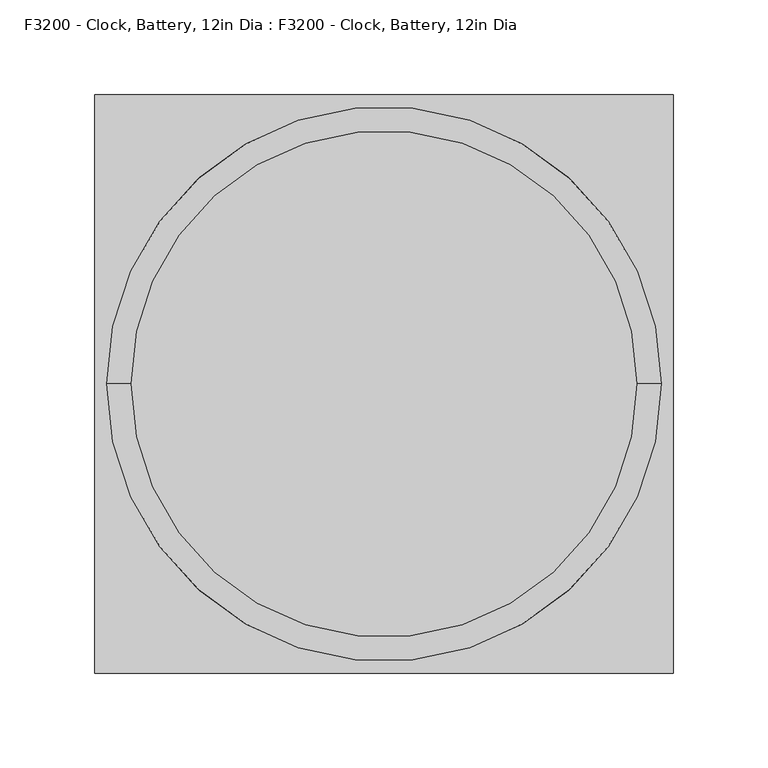
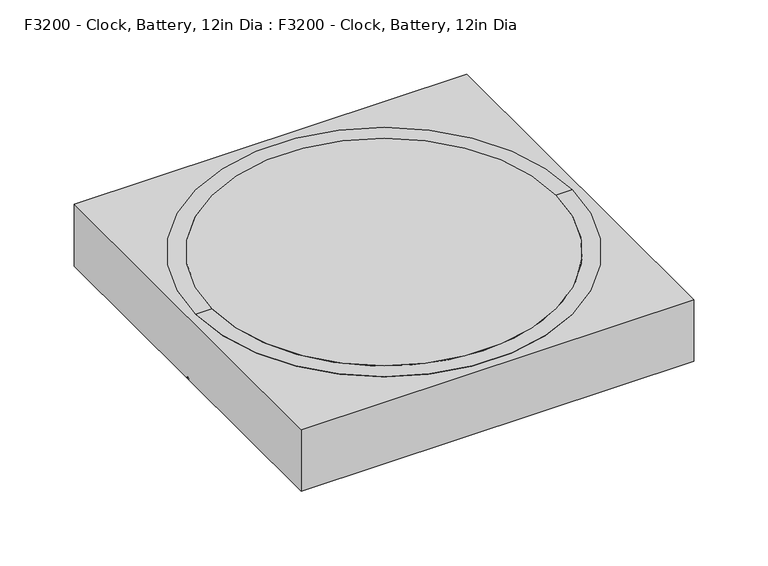
"""IFC4 building model written with IfcOpenShell, lengths in millimetres: proxy geometry, F3200 - Clock, Battery, 12in Dia : F3200 - Clock, Battery, 12in Dia."""

import ifcopenshell
import ifcopenshell.guid

model = None  # the IFC model being written
_history = None  # IfcOwnerHistory: only IFC2X3 demands one
_inside = {}  # id of a spatial element -> (the spatial element, [elements in it])
_under = {}  # id of a project, library or spatial element -> (it, [spatial elements below it])
_declared = {}  # id of a project -> (the project, [libraries it declares])
_typed = {}  # id of a type object -> (the type object, [elements of that type])
_made_of = {}  # id of a material, layer set ... -> (it, [elements and type objects made of it])


def new_model(schema):
    """Start an empty IFC model of exactly this schema.

    Asked for "IFC4X3", IfcOpenShell would pick the latest addendum, in which some entities
    have other attributes; the version numbers below select the first issue.
    IFC2X3 requires an IfcOwnerHistory on every rooted entity: one is made here for all.
    """
    global model, _history
    if schema == "IFC4X3":
        model = ifcopenshell.file(schema_version=(4, 3, 0, 0))
    else:
        model = ifcopenshell.file(schema=schema)
    _inside.clear()
    _under.clear()
    _declared.clear()
    _typed.clear()
    _made_of.clear()
    _history = None
    if model.schema == "IFC2X3":
        org = make("IfcOrganization", Name="unknown")
        user = make(
            "IfcPersonAndOrganization",
            ThePerson=make("IfcPerson", FamilyName="unknown"),
            TheOrganization=org,
        )
        app = make(
            "IfcApplication",
            ApplicationDeveloper=org,
            Version="unknown",
            ApplicationFullName="unknown",
            ApplicationIdentifier="unknown",
        )
        _history = make(
            "IfcOwnerHistory",
            OwningUser=user,
            OwningApplication=app,
            ChangeAction="ADDED",
            CreationDate=0,
        )
    return model


def make(cls, **values):
    """One entity of the class cls with the attributes given. An attribute that is None is left unset."""
    return model.create_entity(
        cls, **{name: value for name, value in values.items() if value is not None}
    )


def rooted(cls, **values):
    """An entity with a GlobalId (a new one), such as an element, a storey or a relation."""
    return make(cls, GlobalId=ifcopenshell.guid.new(), OwnerHistory=_history, **values)


def si_unit(unit_type, name, prefix=None):
    """IfcSIUnit, for example si_unit("LENGTHUNIT", "METRE", prefix="MILLI")."""
    return make("IfcSIUnit", UnitType=unit_type, Prefix=prefix, Name=name)


def assignment(units):
    """IfcUnitAssignment: the units of a project."""
    return None if units is None else make("IfcUnitAssignment", Units=units)


def point(xyz):
    """IfcCartesianPoint."""
    return None if xyz is None else make("IfcCartesianPoint", Coordinates=xyz)


def direction(xyz):
    """IfcDirection."""
    return None if xyz is None else make("IfcDirection", DirectionRatios=xyz)


def frame(location, z_axis=None, x_axis=None):
    """IfcAxis2Placement3D, a coordinate frame: its origin and axes. An axis left out is left unset."""
    return make(
        "IfcAxis2Placement3D",
        Location=point(location),
        Axis=direction(z_axis),
        RefDirection=direction(x_axis),
    )


def frame_2d(location, x_axis=None):
    """IfcAxis2Placement2D, a coordinate frame in the plane: its origin and x axis."""
    return make(
        "IfcAxis2Placement2D", Location=point(location), RefDirection=direction(x_axis)
    )


def origin():
    """The frame at (0, 0, 0) with its axes left unset."""
    return frame((0.0, 0.0, 0.0))


def origin_with_axes():
    """The frame at (0, 0, 0) with the z axis (0, 0, 1) and the x axis (1, 0, 0) written out."""
    return frame((0.0, 0.0, 0.0), z_axis=(0.0, 0.0, 1.0), x_axis=(1.0, 0.0, 0.0))


def place(relative_to, where):
    """IfcLocalPlacement: puts the frame where relative to a parent placement (None: the world)."""
    return make(
        "IfcLocalPlacement", PlacementRelTo=relative_to, RelativePlacement=where
    )


def context(
    kind, dimensions, precision=None, world=None, true_north=None, identifier=None
):
    """IfcGeometricRepresentationContext, for example the 3D "Model" context."""
    return make(
        "IfcGeometricRepresentationContext",
        ContextIdentifier=identifier,
        ContextType=kind,
        CoordinateSpaceDimension=dimensions,
        Precision=precision,
        WorldCoordinateSystem=world,
        TrueNorth=true_north,
    )


def project(units=None, contexts=None):
    """IfcProject with its units and contexts."""
    return rooted(
        "IfcProject",
        Name="project",
        RepresentationContexts=contexts,
        UnitsInContext=assignment(units),
    )


def spatial(cls, under=None, at=None, **own):
    """A site, building, storey or space (cls), placed at a placement, below another one or the project."""
    s = rooted(cls, ObjectPlacement=at, **own)
    if under is not None:
        _under.setdefault(under.id(), (under, []))[1].append(s)
    return s


def polyline(points):
    """IfcPolyline through the points."""
    return make("IfcPolyline", Points=[point(p) for p in points])


def circle_curve(where, radius):
    """IfcCircle in the frame where."""
    return make("IfcCircle", Position=where, Radius=radius)


def trimmed(basis, trim1, trim2, sense, master):
    """IfcTrimmedCurve: the piece of a basis curve between two trims."""
    return make(
        "IfcTrimmedCurve",
        BasisCurve=basis,
        Trim1=trim1,
        Trim2=trim2,
        SenseAgreement=sense,
        MasterRepresentation=master,
    )


def segment(curve, same_sense, transition):
    """IfcCompositeCurveSegment."""
    return make(
        "IfcCompositeCurveSegment",
        Transition=transition,
        SameSense=same_sense,
        ParentCurve=curve,
    )


def composite_curve(segments, self_intersect=None):
    """IfcCompositeCurve: segments joined end to end."""
    return make("IfcCompositeCurve", Segments=segments, SelfIntersect=self_intersect)


def outline(outer, holes=None, kind="AREA"):
    """IfcArbitraryClosedProfileDef: a profile drawn as a closed curve; with holes, ...WithVoids."""
    if holes is None:
        return make("IfcArbitraryClosedProfileDef", ProfileType=kind, OuterCurve=outer)
    return make(
        "IfcArbitraryProfileDefWithVoids",
        ProfileType=kind,
        OuterCurve=outer,
        InnerCurves=holes,
    )


def extrude(swept, where, along, depth):
    """IfcExtrudedAreaSolid: the profile swept, set in the frame where, extruded along a direction by depth."""
    return make(
        "IfcExtrudedAreaSolid",
        SweptArea=swept,
        Position=where,
        ExtrudedDirection=direction(along),
        Depth=depth,
    )


def shape(context_of_items, identifier, shape_type, items):
    """IfcShapeRepresentation: the items that make up one representation, for example the "Body"."""
    return make(
        "IfcShapeRepresentation",
        ContextOfItems=context_of_items,
        RepresentationIdentifier=identifier,
        RepresentationType=shape_type,
        Items=items,
    )


def source(mapping_origin, context_of_items, identifier, shape_type, items):
    """IfcRepresentationMap: a shape defined once, which mapped items show again and again."""
    return make(
        "IfcRepresentationMap",
        MappingOrigin=mapping_origin,
        MappedRepresentation=shape(context_of_items, identifier, shape_type, items),
    )


def transform(
    local_origin,
    x_axis=None,
    y_axis=None,
    z_axis=None,
    scale=None,
    scale2=None,
    scale3=None,
    uniform=True,
):
    """IfcCartesianTransformationOperator3D, or its non-uniform kind. x_axis, y_axis, z_axis: its Axis1, 2, 3."""
    if uniform:
        return make(
            "IfcCartesianTransformationOperator3D",
            Axis1=direction(x_axis),
            Axis2=direction(y_axis),
            LocalOrigin=point(local_origin),
            Scale=scale,
            Axis3=direction(z_axis),
        )
    return make(
        "IfcCartesianTransformationOperator3DnonUniform",
        Axis1=direction(x_axis),
        Axis2=direction(y_axis),
        LocalOrigin=point(local_origin),
        Scale=scale,
        Axis3=direction(z_axis),
        Scale2=scale2,
        Scale3=scale3,
    )


def mapped(mapping_source, mapping_target):
    """IfcMappedItem: shows the shape of a source again, moved by a transform."""
    return make(
        "IfcMappedItem", MappingSource=mapping_source, MappingTarget=mapping_target
    )


def made_of(thing, what):
    """Note that an element or type object is made of a material, layer set ...; save() writes the relation."""
    if what is not None:
        _made_of.setdefault(what.id(), (what, []))[1].append(thing)
    return thing


def element(
    cls,
    number,
    at=None,
    inside=None,
    cuts=None,
    type_object=None,
    material=None,
    context=None,
    identifier="Body",
    shape_type=None,
    held_by="IfcProductDefinitionShape",
    body=None,
    shapes=None,
    **own,
):
    """One element of the class cls, such as IfcWall. Its Tag is "e" and its number.

    at: its placement. inside: the storey or other place that contains it. cuts: it is an
    opening in that element (IfcRelVoidsElement). A single representation is given by context,
    identifier, shape_type and body (its items); several are given by shapes. held_by: the class
    of the entity that holds the representations. save() writes the other relations.
    """
    e = rooted(cls, Tag="e%d" % number, ObjectPlacement=at, **own)
    if body is not None:
        shapes = [shape(context, identifier, shape_type, body)]
    if shapes is not None:
        e.Representation = make(held_by, Representations=shapes)
    if inside is not None:
        _inside.setdefault(inside.id(), (inside, []))[1].append(e)
    if cuts is not None:
        rooted(
            "IfcRelVoidsElement", RelatingBuildingElement=cuts, RelatedOpeningElement=e
        )
    if type_object is not None:
        _typed.setdefault(type_object.id(), (type_object, []))[1].append(e)
    return made_of(e, material)


def aggregate(whole, parts):
    """IfcRelAggregates: a whole, such as a stair, and the parts it consists of."""
    return rooted("IfcRelAggregates", RelatingObject=whole, RelatedObjects=parts)


def save(model, path):
    """Write the relations noted so far, then the file.

    IfcRelAggregates (storeys below a building ...), IfcRelContainedInSpatialStructure (elements
    in a storey), IfcRelDefinesByType, IfcRelAssociatesMaterial and IfcRelDeclares: one each for
    every whole, place, type object, material and project.
    """
    for whole, parts in _under.values():
        aggregate(whole, parts)
    for where, things in _inside.values():
        rooted(
            "IfcRelContainedInSpatialStructure",
            RelatedElements=things,
            RelatingStructure=where,
        )
    for kind, things in _typed.values():
        rooted("IfcRelDefinesByType", RelatedObjects=things, RelatingType=kind)
    for what, things in _made_of.values():
        rooted("IfcRelAssociatesMaterial", RelatedObjects=things, RelatingMaterial=what)
    for by, libraries in _declared.values():
        rooted("IfcRelDeclares", RelatingContext=by, RelatedDefinitions=libraries)
    model.write(path)


def plane_surface(at):
    """IfcPlane: the flat surface through the origin of the frame at, square to its z axis."""
    return make("IfcPlane", Position=at)


def revolved_surface(curve, axis_point, axis_direction):
    """IfcSurfaceOfRevolution: the curve turned about the line through axis_point along axis_direction."""
    return make(
        "IfcSurfaceOfRevolution",
        SweptCurve=make("IfcArbitraryOpenProfileDef", ProfileType="CURVE", Curve=curve),
        AxisPosition=make("IfcAxis1Placement", Location=point(axis_point), Axis=direction(axis_direction)),
    )


def advanced_brep(points, edges, surfaces, faces):
    """IfcAdvancedBrep: a solid bounded by faces that lie on surfaces and meet in shared edges.

    An edge is (start, end): straight between two places in points (the first is 0);
    or (start, end, curve); or (start, end, curve, False) where it runs against its curve.
    A face is (place in surfaces, loops), or (place, loops, False) where it looks against
    its surface's normal. A loop lists edges by number (the first is 1), with a minus sign
    where the edge is run from its end to its start. The first loop is the outer one.
    """
    corners = [point(p) for p in points]
    vertices = [make("IfcVertexPoint", VertexGeometry=c) for c in corners]
    made = []
    for start, end, *more in edges:
        made.append(
            make(
                "IfcEdgeCurve",
                EdgeStart=vertices[start],
                EdgeEnd=vertices[end],
                EdgeGeometry=more[0] if more else make("IfcPolyline", Points=[corners[start], corners[end]]),
                SameSense=more[1] if len(more) > 1 else True,
            )
        )
    hull = []
    for where, loops, *sense in faces:
        bounds = []
        for j, loop in enumerate(loops):
            ring = [make("IfcOrientedEdge", EdgeElement=made[abs(k) - 1], Orientation=k > 0) for k in loop]
            bounds.append(
                make(
                    "IfcFaceOuterBound" if j == 0 else "IfcFaceBound",
                    Bound=make("IfcEdgeLoop", EdgeList=ring),
                    Orientation=True,
                )
            )
        hull.append(make("IfcAdvancedFace", Bounds=bounds, FaceSurface=surfaces[where], SameSense=sense[0] if sense else True))
    return make("IfcAdvancedBrep", Outer=make("IfcClosedShell", CfsFaces=hull))


def f3200_clock_battery_12in_dia_f3200_clock_battery_12in_dia_a6ed2e24(model_context):
    return source(origin(), model_context, "Body", "SolidModel", [
        extrude(outline(composite_curve([segment(trimmed(circle_curve(frame_2d((0.0, 152.4)), 133.35), [point((-133.35, 152.4))], [point((133.35, 152.4))], False, "CARTESIAN"), True, "CONTINUOUS"), segment(trimmed(circle_curve(frame_2d((0.0, 152.4)), 133.35), [point((133.35, 152.4))], [point((-133.35, 152.4))], False, "CARTESIAN"), True, "CONTINUOUS")], self_intersect=False)), frame((0.0, 0.0, 44.45), z_axis=(0.0, 0.0, 1.0), x_axis=(1.0, 0.0, 0.0)), (0.0, 0.0, 1.0), 6.35),
        advanced_brep(
        [(0.0, 152.4, 0.0), (152.4, 152.4, 0.0), (-152.4, 152.4, 0.0), (-133.35, 152.4, 44.45), (133.35, 152.4, 44.45), (0.0, 152.4, 44.45), (-133.35, 152.4, 50.8), (133.35, 152.4, 50.8), (-146.05, 152.4, 50.8), (146.05, 152.4, 50.8)],
        [
            (0, 1),
            (1, 2, circle_curve(frame((0.0, 152.4, 0.0), z_axis=(0.0, 0.0, -1.0), x_axis=(1.0, 0.0, 0.0)), 152.4)),
            (2, 0),
            (2, 1, circle_curve(frame((0.0, 152.4, 0.0), z_axis=(0.0, 0.0, -1.0), x_axis=(1.0, 0.0, 0.0)), 152.4)),
            (3, 4, circle_curve(frame((0.0, 152.4, 44.45), z_axis=(0.0, 0.0, 1.0), x_axis=(1.0, 0.0, 0.0)), 133.35)),
            (4, 5),
            (5, 3),
            (4, 3, circle_curve(frame((0.0, 152.4, 44.45), z_axis=(0.0, 0.0, 1.0), x_axis=(1.0, 0.0, 0.0)), 133.35)),
            (6, 7, circle_curve(frame((0.0, 152.4, 50.8), z_axis=(0.0, 0.0, 1.0), x_axis=(1.0, 0.0, 0.0)), 133.35)),
            (7, 4),
            (3, 6),
            (7, 6, circle_curve(frame((0.0, 152.4, 50.8), z_axis=(0.0, 0.0, 1.0), x_axis=(1.0, 0.0, 0.0)), 133.35)),
            (8, 9, circle_curve(frame((0.0, 152.4, 50.8), z_axis=(0.0, 0.0, 1.0), x_axis=(1.0, 0.0, 0.0)), 146.05)),
            (9, 7),
            (6, 8),
            (9, 8, circle_curve(frame((0.0, 152.4, 50.8), z_axis=(0.0, 0.0, 1.0), x_axis=(1.0, 0.0, 0.0)), 146.05)),
            (1, 9),
            (8, 2),
        ],
        [
            plane_surface(frame((0.0, 152.4, 0.0), z_axis=(0.0, 0.0, -1.0), x_axis=(1.0, 0.0, 0.0))),
            plane_surface(frame((0.0, 152.4, 44.45), z_axis=(0.0, 0.0, 1.0), x_axis=(1.0, 0.0, 0.0))),
            revolved_surface(polyline([(133.35, 152.4, 44.45), (133.35, 152.4, 50.8)]), (0.0, 152.4, 0.0), (0.0, 0.0, -1.0)),
            plane_surface(frame((0.0, 152.4, 50.8), z_axis=(0.0, 0.0, 1.0), x_axis=(1.0, 0.0, 0.0))),
            revolved_surface(polyline([(146.05, 152.4, 50.8), (152.4, 152.4, 0.0)]), (0.0, 152.4, 0.0), (0.0, 0.0, -1.0)),
        ],
        [
            (0, [[1, 2, 3]]),
            (0, [[-3, 4, -1]]),
            (1, [[5, 6, 7]]),
            (1, [[8, -7, -6]]),
            (2, [[9, 10, -5, 11]]),
            (2, [[12, -11, -8, -10]]),
            (3, [[13, 14, -9, 15]]),
            (3, [[16, -15, -12, -14]]),
            (4, [[-2, 17, -13, 18]]),
            (4, [[-4, -18, -16, -17]]),
        ],
    ),
        extrude(outline(polyline([(152.4, 304.8), (152.4, 0.0), (-152.4, 0.0), (-152.4, 304.8), (152.4, 304.8)])), origin_with_axes(), (0.0, 0.0, 1.0), 50.8),
    ])


if __name__ == "__main__":
    model = new_model("IFC4")
    model_context = context("Model", 3, world=origin())
    ifc_project = project(units=[si_unit("LENGTHUNIT", "METRE", prefix="MILLI")], contexts=[model_context])
    site = spatial("IfcSite", under=ifc_project)
    building = spatial("IfcBuilding", under=site)
    placement = place(None, origin())
    f3200_clock_battery_12in_dia_f3200_clock_battery_12in_dia_shape = f3200_clock_battery_12in_dia_f3200_clock_battery_12in_dia_a6ed2e24(model_context)
    element("IfcBuildingElementProxy", 1, Name="F3200 - Clock, Battery, 12in Dia : F3200 - Clock, Battery, 12in Dia", ObjectType="F3200 - Clock, Battery, 12in Dia : F3200 - Clock, Battery, 12in Dia", at=placement, inside=building, context=model_context, shape_type="MappedRepresentation", body=[
        mapped(f3200_clock_battery_12in_dia_f3200_clock_battery_12in_dia_shape, transform((0.0, 0.0, 0.0), x_axis=(1.0, 0.0, 0.0), y_axis=(0.0, 1.0, 0.0), z_axis=(0.0, 0.0, 1.0))),
    ])
    save(model, "model.ifc")

# Revit data of these elements
# Type "F3200 - Clock, Battery, 12in Dia : F3200 - Clock, Battery, 12in Dia"
#   Watts2 = "0"
#   Watts1 = "0"
#   Unit_Issue = "EA"
#   UTIL_6_Misc = "-"
#   UTIL_5_NonMedGas = "-"
#   UTIL_4_MiscGas = "-"
#   UTIL_3_MedGas = "-"
#   UTIL_2_Elec = "-"
#   UTIL_1_WaterDrain = "-"
#   Nomenclature = "Clock, Battery, 12\" Diameter"
#   NSN = "6645"
#   Location [instance default] = ""
#   JSN = "F3200"
#   Fund_Source_VA = "-"
#   Fund_Source_Navy = "-"
#   Fund_Source_Army = "-"
#   Fund_Source_AF = "-"
#   ELEC_Volts2 = "0"
#   ELEC_Volts1 = "0"
#   ELEC_Phase2 = "0"
#   ELEC_Phase1 = "0"
#   ELEC_HertzSwitch = "0"
#   ELEC_HertzDependent = "0"
#   ELEC_Hertz = "0"
#   ELEC_Amps2 = "0"
#   ELEC_Amps1 = "0"
#   DetailDescription = "Clock, 12\" diameter. Round surface, easy to read numbers with sweep second hand. Wall mounted unit for use when impractical to install a fully synchronized clock system. Battery operated, (batteries not included)."
#   CAT_VA = "C"
#   CAT_Navy = "C"
#   CAT_IHS = "-"
#   CAT_Army = "C"
#   CAT_AF = "C"
#   BTUperhour = "0"
#   radius = 0' - 6"
#   Weight_IP = 2
#   Default Elevation = 6' - 6"
#   DIM_Width_IP = 1' - 0"
#   DIM_Height_IP = 1' - 0"
#   DIM_Depth_IP = 0' - 2"
#   Assembly Code = ""
# Element 1 (IfcBuildingElementProxy, "F3200 - Clock, Battery, 12in Dia : F3200 - Clock, Battery, 12in Dia")
#   Location = "ORGS1"
#   Materials on its faces: "EquipSpace", "White"
# Materials
#   "EquipSpace": class "Unassigned", colour RGB 221 217 195, transparency 0.5
#   "White": class "Miscellaneous", colour RGB 255 255 255, transparency 0.4
